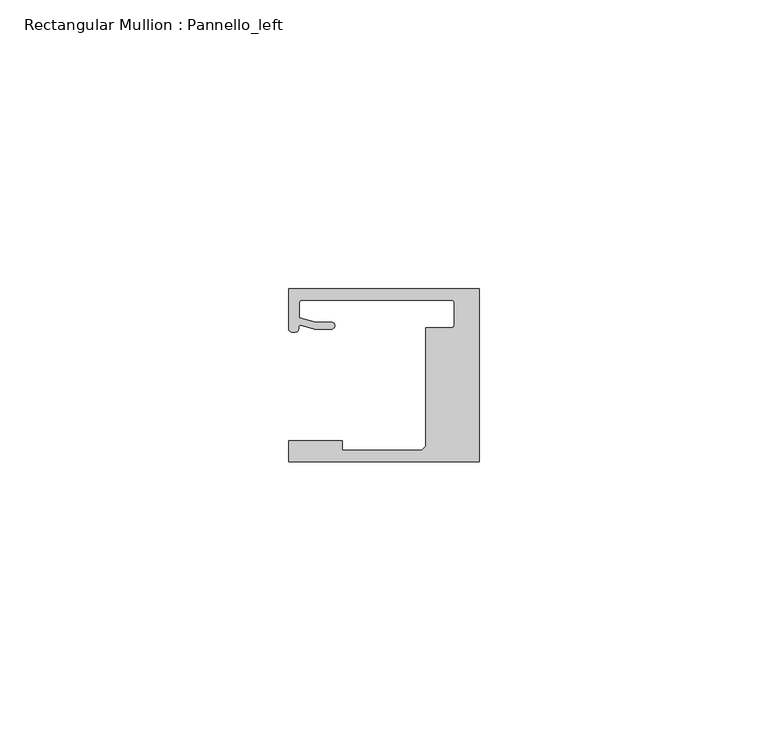
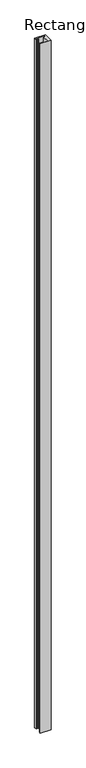
"""IFC4 building model written with IfcOpenShell, lengths in millimetres: member geometry, Rectangular Mullion : Pannello_left."""

from ifc_helpers import new_model, si_unit, frame, origin, place, context, project, spatial, polyline, circle_curve, source, transform, mapped, element, save
from ifc_brep_helpers import plane_surface, cylinder_surface, revolved_surface, extruded_surface, spline_curve, advanced_brep


def rectangular_mullion_pannello_left_fbf18d63(model_context):
    return source(origin(), model_context, "Body", "AdvancedBrep", [
        advanced_brep(
        [(-33.0, -15.0, 0.0), (0.0, -15.0, 0.0), (0.0, 15.0, 0.0), (-33.0000135, 15.0, 0.0), (-33.0000135, 8.0000472, 0.0), (-30.9223017, 8.6490241, 0.0), (-28.4999305, 7.9999523, 0.0), (-25.59998, 7.9999523, 0.0), (-25.59998, 9.1999523, 0.0), (-28.3419477, 9.1999523, 0.0), (-31.19998, 9.9657591, 0.0), (-31.19998, 12.50001, 0.0), (-30.69998, 13.00001, 0.0), (-4.7999726, 13.00001, 0.0), (-4.2999726, 12.50001, 0.0), (-4.2999726, 8.7500595, 0.0), (-4.7999726, 8.2500595, 0.0), (-9.2999726, 8.2500595, 0.0), (-9.2999726, -12.2999849, 0.0), (-10.0000103, -13.0000004, 0.0), (-23.700041, -13.0000004, 0.0), (-23.700041, -11.3000004, 0.0), (-33.0, -11.3000004, 0.0), (-33.0, -15.0, -2260.0), (-33.0, -11.3000004, -2260.0), (-23.700041, -11.3000004, -2260.0), (-23.700041, -13.0000004, -2260.0), (-10.0000103, -13.0000004, -2260.0), (-9.2999726, -12.2999849, -2260.0), (-9.2999726, 8.2500595, -2260.0), (-4.7999726, 8.2500595, -2260.0), (-4.2999726, 8.7500595, -2260.0), (-4.2999726, 12.50001, -2260.0), (-4.7999726, 13.00001, -2260.0), (-30.69998, 13.00001, -2260.0), (-31.19998, 12.50001, -2260.0), (-31.19998, 9.9657591, -2260.0), (-28.3419477, 9.1999523, -2260.0), (-25.59998, 9.1999523, -2260.0), (-25.59998, 7.9999523, -2260.0), (-28.4999305, 7.9999523, -2260.0), (-30.9223017, 8.6490241, -2260.0), (-33.0000135, 8.0000472, -2260.0), (-33.0000135, 15.0, -2260.0), (0.0, 15.0, -2260.0), (0.0, -15.0, -2260.0)],
        [
            (0, 1),
            (1, 2),
            (2, 3),
            (3, 4),
            (4, 5, spline_curve(3, [(-33.0000135, 8.0000472, 0.0), (-33.0000135, 7.457047519, 0.0), (-32.262327879, 7.456527435, 0.0), (-31.357433266, 7.563996614, 0.0), (-31.305645054, 7.690065204, 0.0), (-31.298563602, 8.366228555, 0.0), (-31.312054066, 8.717747958, 0.0), (-30.9223017, 8.6490241, 0.0)], [4, 2, 2, 4], [0.0, 0.0027053965905959043, 0.0058611956533709, 0.007702013405570312])),
            (5, 6),
            (6, 7),
            (7, 8, circle_curve(frame((-25.59998, 8.5999523, 0.0), z_axis=(0.0, 0.0, 1.0), x_axis=(0.0, 1.0, 0.0)), 0.6)),
            (8, 9),
            (9, 10),
            (10, 11),
            (11, 12, circle_curve(frame((-30.69998, 12.50001, 0.0), z_axis=(0.0, 0.0, -1.0), x_axis=(0.0, 1.0, 0.0)), 0.5)),
            (12, 13),
            (13, 14, circle_curve(frame((-4.7999726, 12.50001, 0.0), z_axis=(0.0, 0.0, -1.0), x_axis=(1.0, 0.0, 0.0)), 0.5)),
            (14, 15),
            (15, 16, circle_curve(frame((-4.7999726, 8.7500595, 0.0), z_axis=(0.0, 0.0, -1.0), x_axis=(0.0, -1.0, 0.0)), 0.5)),
            (16, 17),
            (17, 18),
            (18, 19),
            (19, 20),
            (20, 21),
            (21, 22),
            (22, 0),
            (23, 24),
            (24, 25),
            (25, 26),
            (26, 27),
            (27, 28),
            (28, 29),
            (29, 30),
            (30, 31, circle_curve(frame((-4.7999726, 8.7500595, -2260.0), z_axis=(0.0, 0.0, 1.0), x_axis=(0.0, -1.0, 0.0)), 0.5)),
            (31, 32),
            (32, 33, circle_curve(frame((-4.7999726, 12.50001, -2260.0), z_axis=(0.0, 0.0, 1.0), x_axis=(1.0, 0.0, 0.0)), 0.5)),
            (33, 34),
            (34, 35, circle_curve(frame((-30.69998, 12.50001, -2260.0), z_axis=(0.0, 0.0, 1.0), x_axis=(0.0, 1.0, 0.0)), 0.5)),
            (35, 36),
            (36, 37),
            (37, 38),
            (38, 39, circle_curve(frame((-25.59998, 8.5999523, -2260.0), z_axis=(0.0, 0.0, -1.0), x_axis=(0.0, 1.0, 0.0)), 0.6)),
            (39, 40),
            (40, 41),
            (41, 42, spline_curve(3, [(-30.9223017, 8.6490241, -2260.0), (-31.312054066, 8.717747958, -2260.0), (-31.298563602, 8.366228555, -2260.0), (-31.305645054, 7.690065204, -2260.0), (-31.357433266, 7.563996614, -2260.0), (-32.262327879, 7.456527435, -2260.0), (-33.0000135, 7.457047519, -2260.0), (-33.0000135, 8.0000472, -2260.0)], [4, 2, 2, 4], [0.0, 0.001840817752199412, 0.004996616814974408, 0.007702013405570312])),
            (42, 43),
            (43, 44),
            (44, 45),
            (45, 23),
            (0, 23),
            (45, 1),
            (44, 2),
            (43, 3),
            (42, 4),
            (41, 5),
            (40, 6),
            (39, 7),
            (38, 8),
            (37, 9),
            (36, 10),
            (35, 11),
            (34, 12),
            (33, 13),
            (32, 14),
            (31, 15),
            (30, 16),
            (29, 17),
            (28, 18),
            (27, 19),
            (26, 20),
            (25, 21),
            (24, 22),
        ],
        [
            plane_surface(frame((0.0, -36.2491502, 0.0), z_axis=(0.0, 0.0, 1.0), x_axis=(-1.0, 0.0, 0.0))),
            plane_surface(frame((0.0, -36.2491502, -2260.0), z_axis=(0.0, 0.0, -1.0), x_axis=(-1.0, 0.0, 0.0))),
            plane_surface(frame((-33.0, -15.0, 0.0), z_axis=(0.0, -1.0, 0.0), x_axis=(0.0, 0.0, -1.0))),
            plane_surface(frame((0.0, -15.0, 0.0), z_axis=(1.0, 0.0, 0.0), x_axis=(0.0, 0.0, -1.0))),
            plane_surface(frame((0.0, 15.0, 0.0), z_axis=(0.0, 1.0, 0.0), x_axis=(0.0, 0.0, -1.0))),
            plane_surface(frame((-33.0000135, 15.0, 0.0), z_axis=(-1.0, 0.0, 0.0), x_axis=(0.0, 0.0, -1.0))),
            extruded_surface(spline_curve(3, [(-33.0000135, 8.0000472, -2260.0), (-33.0000135, 7.457047519, -2260.0), (-32.262327879, 7.456527435, -2260.0), (-31.357433266, 7.563996614, -2260.0), (-31.305645054, 7.690065204, -2260.0), (-31.298563602, 8.366228555, -2260.0), (-31.312054066, 8.717747958, -2260.0), (-30.9223017, 8.6490241, -2260.0)], [4, 2, 2, 4], [0.0, 0.0027053965905959043, 0.0058611956533709, 0.007702013405570312]), (0.0, 0.0, 2260.0), 2260.0),
            plane_surface(frame((-30.9223017, 8.6490241, 0.0), z_axis=(-0.25881883200192934, -0.9659258833891746, 0.0), x_axis=(0.0, 0.0, -1.0))),
            plane_surface(frame((-28.4999305, 7.9999523, 0.0), z_axis=(0.0, -1.0, 0.0), x_axis=(0.0, 0.0, -1.0))),
            cylinder_surface(frame((-25.59998, 8.5999523, 0.0), z_axis=(0.0, 0.0, 1.0), x_axis=(0.0, 1.0, 0.0)), 0.6),
            plane_surface(frame((-25.59998, 9.1999523, 0.0), z_axis=(0.0, 1.0, 0.0), x_axis=(0.0, 0.0, -1.0))),
            plane_surface(frame((-28.3419477, 9.1999523, 0.0), z_axis=(0.25881883204288636, 0.9659258833782002, 0.0), x_axis=(0.0, 0.0, -1.0))),
            plane_surface(frame((-31.19998, 9.9657591, 0.0), z_axis=(1.0, 0.0, 0.0), x_axis=(0.0, 0.0, -1.0))),
            revolved_surface(polyline([(-30.69998, 13.00001, -2260.0), (-30.69998, 13.00001, 0.0)]), (-30.69998, 12.50001, 0.0), (0.0, 0.0, -1.0)),
            plane_surface(frame((-30.69998, 13.00001, 0.0), z_axis=(0.0, -1.0, 0.0), x_axis=(0.0, 0.0, -1.0))),
            revolved_surface(polyline([(-4.2999726, 12.50001, -2260.0), (-4.2999726, 12.50001, 0.0)]), (-4.7999726, 12.50001, 0.0), (0.0, 0.0, -1.0)),
            plane_surface(frame((-4.2999726, 12.50001, 0.0), z_axis=(-1.0, 0.0, 0.0), x_axis=(0.0, 0.0, -1.0))),
            revolved_surface(polyline([(-4.7999726, 8.2500595, -2260.0), (-4.7999726, 8.2500595, 0.0)]), (-4.7999726, 8.7500595, 0.0), (0.0, 0.0, -1.0)),
            plane_surface(frame((-4.7999726, 8.2500595, 0.0), z_axis=(0.0, 1.0, 0.0), x_axis=(0.0, 0.0, -1.0))),
            plane_surface(frame((-9.2999726, 8.2500595, 0.0), z_axis=(-1.0, 0.0, 0.0), x_axis=(0.0, 0.0, -1.0))),
            plane_surface(frame((-9.2999726, -12.2999849, 0.0), z_axis=(-0.7070955486277984, 0.7071180135668678, 0.0), x_axis=(0.0, 0.0, -1.0))),
            plane_surface(frame((-10.0000103, -13.0000004, 0.0), z_axis=(0.0, 1.0, 0.0), x_axis=(0.0, 0.0, -1.0))),
            plane_surface(frame((-23.700041, -13.0000004, 0.0), z_axis=(1.0, 0.0, 0.0), x_axis=(0.0, 0.0, -1.0))),
            plane_surface(frame((-23.700041, -11.3000004, 0.0), z_axis=(0.0, 1.0, 0.0), x_axis=(0.0, 0.0, -1.0))),
            plane_surface(frame((-33.0, -11.3000004, 0.0), z_axis=(-1.0, 0.0, 0.0), x_axis=(0.0, 0.0, -1.0))),
        ],
        [
            (0, [[1, 2, 3, 4, 5, 6, 7, 8, 9, 10, 11, 12, 13, 14, 15, 16, 17, 18, 19, 20, 21, 22, 23]]),
            (1, [[24, 25, 26, 27, 28, 29, 30, 31, 32, 33, 34, 35, 36, 37, 38, 39, 40, 41, 42, 43, 44, 45, 46]]),
            (2, [[-1, 47, -46, 48]]),
            (3, [[-2, -48, -45, 49]]),
            (4, [[-3, -49, -44, 50]]),
            (5, [[-4, -50, -43, 51]]),
            (6, [[-5, -51, -42, 52]]),
            (7, [[-6, -52, -41, 53]]),
            (8, [[-7, -53, -40, 54]]),
            (9, [[-8, -54, -39, 55]]),
            (10, [[-9, -55, -38, 56]]),
            (11, [[-10, -56, -37, 57]]),
            (12, [[-11, -57, -36, 58]]),
            (13, [[-12, -58, -35, 59]]),
            (14, [[-13, -59, -34, 60]]),
            (15, [[-14, -60, -33, 61]]),
            (16, [[-15, -61, -32, 62]]),
            (17, [[-16, -62, -31, 63]]),
            (18, [[-17, -63, -30, 64]]),
            (19, [[-18, -64, -29, 65]]),
            (20, [[-19, -65, -28, 66]]),
            (21, [[-20, -66, -27, 67]]),
            (22, [[-21, -67, -26, 68]]),
            (23, [[-22, -68, -25, 69]]),
            (24, [[-23, -69, -24, -47]]),
        ],
    ),
    ])


if __name__ == "__main__":
    model = new_model("IFC4")
    model_context = context("Model", 3, world=origin())
    ifc_project = project(units=[si_unit("LENGTHUNIT", "METRE", prefix="MILLI")], contexts=[model_context])
    site = spatial("IfcSite", under=ifc_project)
    building = spatial("IfcBuilding", under=site)
    placement = place(None, origin())
    rectangular_mullion_pannello_left_shape = rectangular_mullion_pannello_left_fbf18d63(model_context)
    element("IfcMember", 1, ObjectType="Rectangular Mullion : Pannello_left", at=placement, inside=building, context=model_context, shape_type="MappedRepresentation", body=[
        mapped(rectangular_mullion_pannello_left_shape, transform((0.0, 0.0, 0.0), x_axis=(1.0, 0.0, 0.0), y_axis=(0.0, 1.0, 0.0), z_axis=(0.0, 0.0, 1.0))),
    ])
    save(model, "model.ifc")

# Revit data of these elements
# Type "Rectangular Mullion : Pannello_left"
#   built-in parameter 1007322 = 0.0984252 (stored number, unit not read)
#   built-in parameter 1007320 = 0.0305117 (stored number, unit not read)
